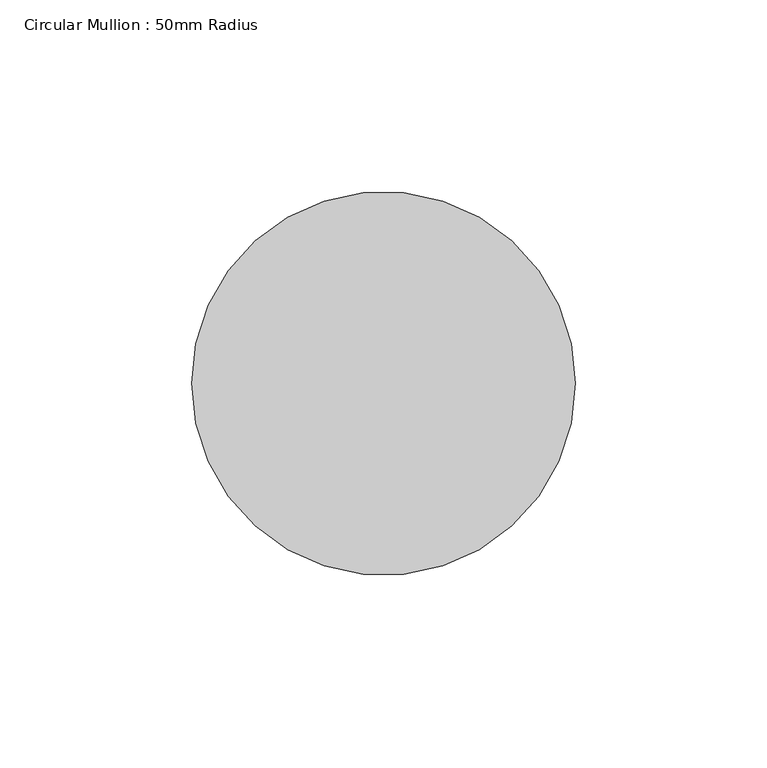
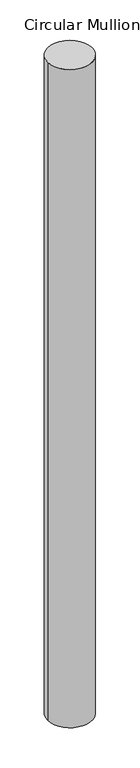
"""IFC4 building model written with IfcOpenShell, lengths in millimetres: member geometry, Circular Mullion : 50mm Radius."""

import ifcopenshell
import ifcopenshell.guid

model = None  # the IFC model being written
_history = None  # IfcOwnerHistory: only IFC2X3 demands one
_inside = {}  # id of a spatial element -> (the spatial element, [elements in it])
_under = {}  # id of a project, library or spatial element -> (it, [spatial elements below it])
_declared = {}  # id of a project -> (the project, [libraries it declares])
_typed = {}  # id of a type object -> (the type object, [elements of that type])
_made_of = {}  # id of a material, layer set ... -> (it, [elements and type objects made of it])


def new_model(schema):
    """Start an empty IFC model of exactly this schema.

    Asked for "IFC4X3", IfcOpenShell would pick the latest addendum, in which some entities
    have other attributes; the version numbers below select the first issue.
    IFC2X3 requires an IfcOwnerHistory on every rooted entity: one is made here for all.
    """
    global model, _history
    if schema == "IFC4X3":
        model = ifcopenshell.file(schema_version=(4, 3, 0, 0))
    else:
        model = ifcopenshell.file(schema=schema)
    _inside.clear()
    _under.clear()
    _declared.clear()
    _typed.clear()
    _made_of.clear()
    _history = None
    if model.schema == "IFC2X3":
        org = make("IfcOrganization", Name="unknown")
        user = make(
            "IfcPersonAndOrganization",
            ThePerson=make("IfcPerson", FamilyName="unknown"),
            TheOrganization=org,
        )
        app = make(
            "IfcApplication",
            ApplicationDeveloper=org,
            Version="unknown",
            ApplicationFullName="unknown",
            ApplicationIdentifier="unknown",
        )
        _history = make(
            "IfcOwnerHistory",
            OwningUser=user,
            OwningApplication=app,
            ChangeAction="ADDED",
            CreationDate=0,
        )
    return model


def make(cls, **values):
    """One entity of the class cls with the attributes given. An attribute that is None is left unset."""
    return model.create_entity(
        cls, **{name: value for name, value in values.items() if value is not None}
    )


def rooted(cls, **values):
    """An entity with a GlobalId (a new one), such as an element, a storey or a relation."""
    return make(cls, GlobalId=ifcopenshell.guid.new(), OwnerHistory=_history, **values)


def si_unit(unit_type, name, prefix=None):
    """IfcSIUnit, for example si_unit("LENGTHUNIT", "METRE", prefix="MILLI")."""
    return make("IfcSIUnit", UnitType=unit_type, Prefix=prefix, Name=name)


def assignment(units):
    """IfcUnitAssignment: the units of a project."""
    return None if units is None else make("IfcUnitAssignment", Units=units)


def point(xyz):
    """IfcCartesianPoint."""
    return None if xyz is None else make("IfcCartesianPoint", Coordinates=xyz)


def direction(xyz):
    """IfcDirection."""
    return None if xyz is None else make("IfcDirection", DirectionRatios=xyz)


def frame(location, z_axis=None, x_axis=None):
    """IfcAxis2Placement3D, a coordinate frame: its origin and axes. An axis left out is left unset."""
    return make(
        "IfcAxis2Placement3D",
        Location=point(location),
        Axis=direction(z_axis),
        RefDirection=direction(x_axis),
    )


def frame_2d(location, x_axis=None):
    """IfcAxis2Placement2D, a coordinate frame in the plane: its origin and x axis."""
    return make(
        "IfcAxis2Placement2D", Location=point(location), RefDirection=direction(x_axis)
    )


def origin():
    """The frame at (0, 0, 0) with its axes left unset."""
    return frame((0.0, 0.0, 0.0))


def origin_2d():
    """The frame at (0, 0) in the plane with its x axis left unset."""
    return frame_2d((0.0, 0.0))


def place(relative_to, where):
    """IfcLocalPlacement: puts the frame where relative to a parent placement (None: the world)."""
    return make(
        "IfcLocalPlacement", PlacementRelTo=relative_to, RelativePlacement=where
    )


def context(
    kind, dimensions, precision=None, world=None, true_north=None, identifier=None
):
    """IfcGeometricRepresentationContext, for example the 3D "Model" context."""
    return make(
        "IfcGeometricRepresentationContext",
        ContextIdentifier=identifier,
        ContextType=kind,
        CoordinateSpaceDimension=dimensions,
        Precision=precision,
        WorldCoordinateSystem=world,
        TrueNorth=true_north,
    )


def project(units=None, contexts=None):
    """IfcProject with its units and contexts."""
    return rooted(
        "IfcProject",
        Name="project",
        RepresentationContexts=contexts,
        UnitsInContext=assignment(units),
    )


def spatial(cls, under=None, at=None, **own):
    """A site, building, storey or space (cls), placed at a placement, below another one or the project."""
    s = rooted(cls, ObjectPlacement=at, **own)
    if under is not None:
        _under.setdefault(under.id(), (under, []))[1].append(s)
    return s


def circle_curve(where, radius):
    """IfcCircle in the frame where."""
    return make("IfcCircle", Position=where, Radius=radius)


def trimmed(basis, trim1, trim2, sense, master):
    """IfcTrimmedCurve: the piece of a basis curve between two trims."""
    return make(
        "IfcTrimmedCurve",
        BasisCurve=basis,
        Trim1=trim1,
        Trim2=trim2,
        SenseAgreement=sense,
        MasterRepresentation=master,
    )


def segment(curve, same_sense, transition):
    """IfcCompositeCurveSegment."""
    return make(
        "IfcCompositeCurveSegment",
        Transition=transition,
        SameSense=same_sense,
        ParentCurve=curve,
    )


def composite_curve(segments, self_intersect=None):
    """IfcCompositeCurve: segments joined end to end."""
    return make("IfcCompositeCurve", Segments=segments, SelfIntersect=self_intersect)


def outline(outer, holes=None, kind="AREA"):
    """IfcArbitraryClosedProfileDef: a profile drawn as a closed curve; with holes, ...WithVoids."""
    if holes is None:
        return make("IfcArbitraryClosedProfileDef", ProfileType=kind, OuterCurve=outer)
    return make(
        "IfcArbitraryProfileDefWithVoids",
        ProfileType=kind,
        OuterCurve=outer,
        InnerCurves=holes,
    )


def extrude(swept, where, along, depth):
    """IfcExtrudedAreaSolid: the profile swept, set in the frame where, extruded along a direction by depth."""
    return make(
        "IfcExtrudedAreaSolid",
        SweptArea=swept,
        Position=where,
        ExtrudedDirection=direction(along),
        Depth=depth,
    )


def shape(context_of_items, identifier, shape_type, items):
    """IfcShapeRepresentation: the items that make up one representation, for example the "Body"."""
    return make(
        "IfcShapeRepresentation",
        ContextOfItems=context_of_items,
        RepresentationIdentifier=identifier,
        RepresentationType=shape_type,
        Items=items,
    )


def source(mapping_origin, context_of_items, identifier, shape_type, items):
    """IfcRepresentationMap: a shape defined once, which mapped items show again and again."""
    return make(
        "IfcRepresentationMap",
        MappingOrigin=mapping_origin,
        MappedRepresentation=shape(context_of_items, identifier, shape_type, items),
    )


def transform(
    local_origin,
    x_axis=None,
    y_axis=None,
    z_axis=None,
    scale=None,
    scale2=None,
    scale3=None,
    uniform=True,
):
    """IfcCartesianTransformationOperator3D, or its non-uniform kind. x_axis, y_axis, z_axis: its Axis1, 2, 3."""
    if uniform:
        return make(
            "IfcCartesianTransformationOperator3D",
            Axis1=direction(x_axis),
            Axis2=direction(y_axis),
            LocalOrigin=point(local_origin),
            Scale=scale,
            Axis3=direction(z_axis),
        )
    return make(
        "IfcCartesianTransformationOperator3DnonUniform",
        Axis1=direction(x_axis),
        Axis2=direction(y_axis),
        LocalOrigin=point(local_origin),
        Scale=scale,
        Axis3=direction(z_axis),
        Scale2=scale2,
        Scale3=scale3,
    )


def mapped(mapping_source, mapping_target):
    """IfcMappedItem: shows the shape of a source again, moved by a transform."""
    return make(
        "IfcMappedItem", MappingSource=mapping_source, MappingTarget=mapping_target
    )


def made_of(thing, what):
    """Note that an element or type object is made of a material, layer set ...; save() writes the relation."""
    if what is not None:
        _made_of.setdefault(what.id(), (what, []))[1].append(thing)
    return thing


def element(
    cls,
    number,
    at=None,
    inside=None,
    cuts=None,
    type_object=None,
    material=None,
    context=None,
    identifier="Body",
    shape_type=None,
    held_by="IfcProductDefinitionShape",
    body=None,
    shapes=None,
    **own,
):
    """One element of the class cls, such as IfcWall. Its Tag is "e" and its number.

    at: its placement. inside: the storey or other place that contains it. cuts: it is an
    opening in that element (IfcRelVoidsElement). A single representation is given by context,
    identifier, shape_type and body (its items); several are given by shapes. held_by: the class
    of the entity that holds the representations. save() writes the other relations.
    """
    e = rooted(cls, Tag="e%d" % number, ObjectPlacement=at, **own)
    if body is not None:
        shapes = [shape(context, identifier, shape_type, body)]
    if shapes is not None:
        e.Representation = make(held_by, Representations=shapes)
    if inside is not None:
        _inside.setdefault(inside.id(), (inside, []))[1].append(e)
    if cuts is not None:
        rooted(
            "IfcRelVoidsElement", RelatingBuildingElement=cuts, RelatedOpeningElement=e
        )
    if type_object is not None:
        _typed.setdefault(type_object.id(), (type_object, []))[1].append(e)
    return made_of(e, material)


def aggregate(whole, parts):
    """IfcRelAggregates: a whole, such as a stair, and the parts it consists of."""
    return rooted("IfcRelAggregates", RelatingObject=whole, RelatedObjects=parts)


def save(model, path):
    """Write the relations noted so far, then the file.

    IfcRelAggregates (storeys below a building ...), IfcRelContainedInSpatialStructure (elements
    in a storey), IfcRelDefinesByType, IfcRelAssociatesMaterial and IfcRelDeclares: one each for
    every whole, place, type object, material and project.
    """
    for whole, parts in _under.values():
        aggregate(whole, parts)
    for where, things in _inside.values():
        rooted(
            "IfcRelContainedInSpatialStructure",
            RelatedElements=things,
            RelatingStructure=where,
        )
    for kind, things in _typed.values():
        rooted("IfcRelDefinesByType", RelatedObjects=things, RelatingType=kind)
    for what, things in _made_of.values():
        rooted("IfcRelAssociatesMaterial", RelatedObjects=things, RelatingMaterial=what)
    for by, libraries in _declared.values():
        rooted("IfcRelDeclares", RelatingContext=by, RelatedDefinitions=libraries)
    model.write(path)


def circular_mullion_50mm_radius_309c7a25(model_context):
    return source(origin(), model_context, "Body", "SweptSolid", [
        extrude(outline(composite_curve([segment(trimmed(circle_curve(origin_2d(), 50.0), [point((50.0, 0.0))], [point((-50.0, 0.0))], False, "CARTESIAN"), True, "CONTINUOUS"), segment(trimmed(circle_curve(origin_2d(), 50.0), [point((-50.0, 0.0))], [point((50.0, 0.0))], False, "CARTESIAN"), True, "CONTINUOUS")], self_intersect=False)), frame((0.0, 0.0, -1569.2846644), z_axis=(0.0, 0.0, 1.0), x_axis=(1.0, 0.0, 0.0)), (0.0, 0.0, 1.0), 1569.2846644),
    ])


if __name__ == "__main__":
    model = new_model("IFC4")
    model_context = context("Model", 3, world=origin())
    ifc_project = project(units=[si_unit("LENGTHUNIT", "METRE", prefix="MILLI")], contexts=[model_context])
    site = spatial("IfcSite", under=ifc_project)
    building = spatial("IfcBuilding", under=site)
    placement = place(None, origin())
    circular_mullion_50mm_radius_shape = circular_mullion_50mm_radius_309c7a25(model_context)
    element("IfcMember", 1, ObjectType="Circular Mullion : 50mm Radius", at=placement, inside=building, context=model_context, shape_type="MappedRepresentation", body=[
        mapped(circular_mullion_50mm_radius_shape, transform((0.0, 0.0, 0.0), x_axis=(1.0, 0.0, 0.0), y_axis=(0.0, 1.0, 0.0), z_axis=(0.0, 0.0, 1.0))),
    ])
    save(model, "model.ifc")

# Revit data of these elements
# Type "Circular Mullion : 50mm Radius"
#   built-in parameter 1007350 = 0.164042 (stored number, unit not read)
# Element 1 (IfcMember, "Circular Mullion : 50mm Radius")
#   Materials on its faces: "Aluminium"
# Materials
#   "Aluminium": class "Metal", colour RGB 247 247 247, transparency 0, Description = "Aluminium 6061", Cost = 0
